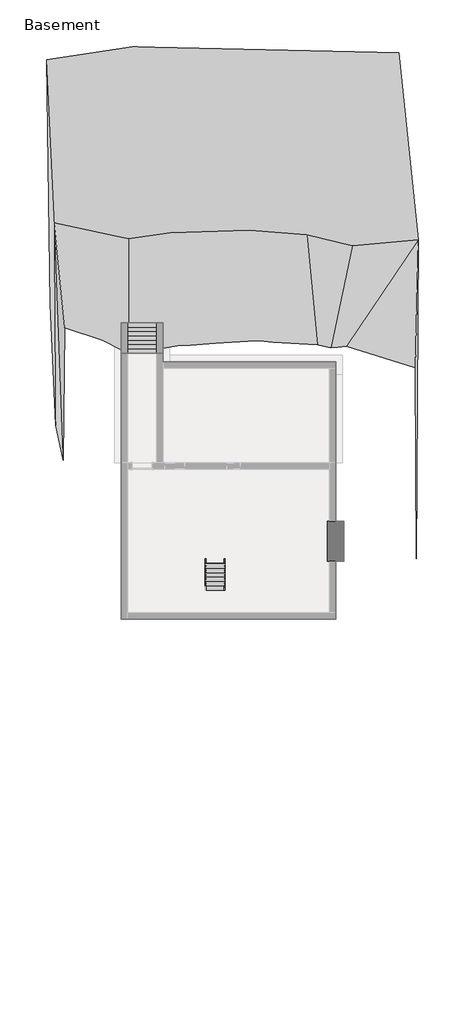
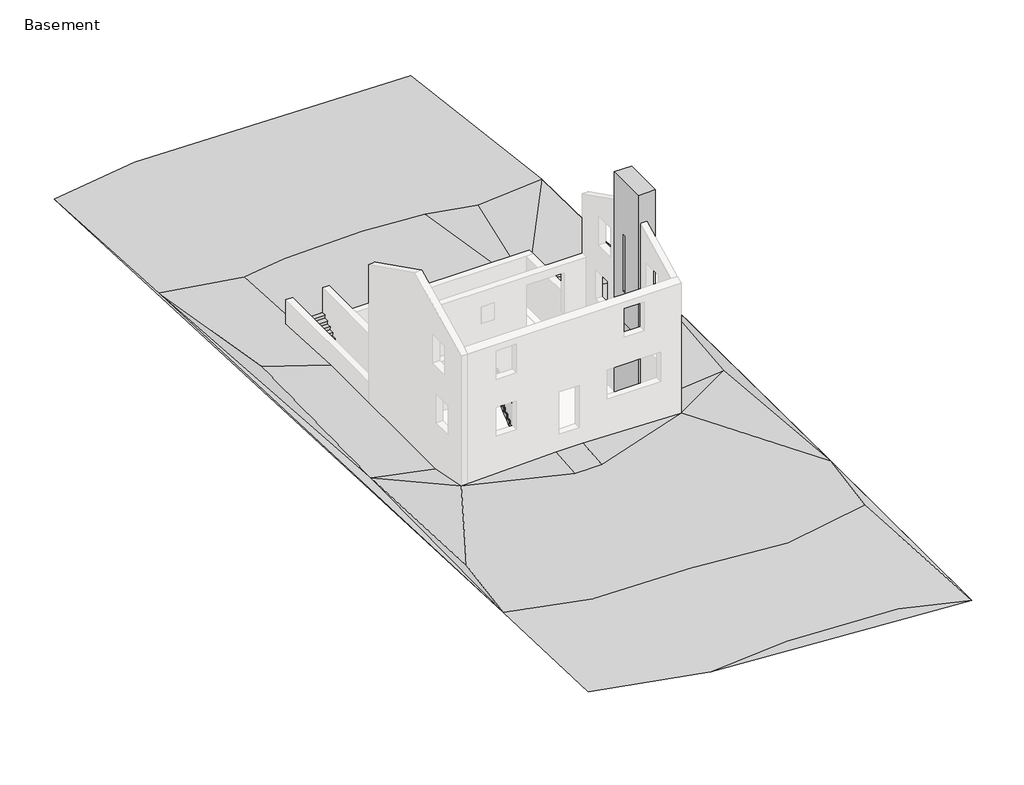
# One storey, part 2 of 2: 5 proxies, 2 members, 2 stair flights, 1 railing.
"""IFC4 building model written with IfcOpenShell, lengths in millimetres."""

import ifcopenshell
import ifcopenshell.guid

model = None  # the IFC model being written
_history = None  # IfcOwnerHistory: only IFC2X3 demands one
_inside = {}  # id of a spatial element -> (the spatial element, [elements in it])
_under = {}  # id of a project, library or spatial element -> (it, [spatial elements below it])
_declared = {}  # id of a project -> (the project, [libraries it declares])
_typed = {}  # id of a type object -> (the type object, [elements of that type])
_made_of = {}  # id of a material, layer set ... -> (it, [elements and type objects made of it])


def new_model(schema):
    """Start an empty IFC model of exactly this schema.

    Asked for "IFC4X3", IfcOpenShell would pick the latest addendum, in which some entities
    have other attributes; the version numbers below select the first issue.
    IFC2X3 requires an IfcOwnerHistory on every rooted entity: one is made here for all.
    """
    global model, _history
    if schema == "IFC4X3":
        model = ifcopenshell.file(schema_version=(4, 3, 0, 0))
    else:
        model = ifcopenshell.file(schema=schema)
    _inside.clear()
    _under.clear()
    _declared.clear()
    _typed.clear()
    _made_of.clear()
    _history = None
    if model.schema == "IFC2X3":
        org = make("IfcOrganization", Name="unknown")
        user = make(
            "IfcPersonAndOrganization",
            ThePerson=make("IfcPerson", FamilyName="unknown"),
            TheOrganization=org,
        )
        app = make(
            "IfcApplication",
            ApplicationDeveloper=org,
            Version="unknown",
            ApplicationFullName="unknown",
            ApplicationIdentifier="unknown",
        )
        _history = make(
            "IfcOwnerHistory",
            OwningUser=user,
            OwningApplication=app,
            ChangeAction="ADDED",
            CreationDate=0,
        )
    return model


def make(cls, **values):
    """One entity of the class cls with the attributes given. An attribute that is None is left unset."""
    return model.create_entity(
        cls, **{name: value for name, value in values.items() if value is not None}
    )


def rooted(cls, **values):
    """An entity with a GlobalId (a new one), such as an element, a storey or a relation."""
    return make(cls, GlobalId=ifcopenshell.guid.new(), OwnerHistory=_history, **values)


def si_unit(unit_type, name, prefix=None):
    """IfcSIUnit, for example si_unit("LENGTHUNIT", "METRE", prefix="MILLI")."""
    return make("IfcSIUnit", UnitType=unit_type, Prefix=prefix, Name=name)


def assignment(units):
    """IfcUnitAssignment: the units of a project."""
    return None if units is None else make("IfcUnitAssignment", Units=units)


def point(xyz):
    """IfcCartesianPoint."""
    return None if xyz is None else make("IfcCartesianPoint", Coordinates=xyz)


def direction(xyz):
    """IfcDirection."""
    return None if xyz is None else make("IfcDirection", DirectionRatios=xyz)


def frame(location, z_axis=None, x_axis=None):
    """IfcAxis2Placement3D, a coordinate frame: its origin and axes. An axis left out is left unset."""
    return make(
        "IfcAxis2Placement3D",
        Location=point(location),
        Axis=direction(z_axis),
        RefDirection=direction(x_axis),
    )


def origin():
    """The frame at (0, 0, 0) with its axes left unset."""
    return frame((0.0, 0.0, 0.0))


def place(relative_to, where):
    """IfcLocalPlacement: puts the frame where relative to a parent placement (None: the world)."""
    return make(
        "IfcLocalPlacement", PlacementRelTo=relative_to, RelativePlacement=where
    )


def context(
    kind, dimensions, precision=None, world=None, true_north=None, identifier=None
):
    """IfcGeometricRepresentationContext, for example the 3D "Model" context."""
    return make(
        "IfcGeometricRepresentationContext",
        ContextIdentifier=identifier,
        ContextType=kind,
        CoordinateSpaceDimension=dimensions,
        Precision=precision,
        WorldCoordinateSystem=world,
        TrueNorth=true_north,
    )


def project(units=None, contexts=None):
    """IfcProject with its units and contexts."""
    return rooted(
        "IfcProject",
        Name="project",
        RepresentationContexts=contexts,
        UnitsInContext=assignment(units),
    )


def spatial(cls, under=None, at=None, **own):
    """A site, building, storey or space (cls), placed at a placement, below another one or the project."""
    s = rooted(cls, ObjectPlacement=at, **own)
    if under is not None:
        _under.setdefault(under.id(), (under, []))[1].append(s)
    return s


def polyline(points):
    """IfcPolyline through the points."""
    return make("IfcPolyline", Points=[point(p) for p in points])


def point_list(points):
    """IfcCartesianPointList2D or 3D."""
    cls = (
        "IfcCartesianPointList2D" if len(points[0]) == 2 else "IfcCartesianPointList3D"
    )
    return make(cls, CoordList=points)


def outline(outer, holes=None, kind="AREA"):
    """IfcArbitraryClosedProfileDef: a profile drawn as a closed curve; with holes, ...WithVoids."""
    if holes is None:
        return make("IfcArbitraryClosedProfileDef", ProfileType=kind, OuterCurve=outer)
    return make(
        "IfcArbitraryProfileDefWithVoids",
        ProfileType=kind,
        OuterCurve=outer,
        InnerCurves=holes,
    )


def extrude(swept, where, along, depth):
    """IfcExtrudedAreaSolid: the profile swept, set in the frame where, extruded along a direction by depth."""
    return make(
        "IfcExtrudedAreaSolid",
        SweptArea=swept,
        Position=where,
        ExtrudedDirection=direction(along),
        Depth=depth,
    )


def faces_of(points, faces, orient=None, outer=None):
    """IfcFace entities. A face is a list of loops; a loop is a list of indices into points, from 0.

    orient and outer hold one flag for each loop. By default every Orientation is true, the
    first loop of a face is its IfcFaceOuterBound and the others are IfcFaceBound.
    """
    made = []
    for i, loops in enumerate(faces):
        bounds = []
        for j, loop in enumerate(loops):
            is_outer = j == 0 if outer is None else outer[i][j]
            bounds.append(
                make(
                    "IfcFaceOuterBound" if is_outer else "IfcFaceBound",
                    Bound=make("IfcPolyLoop", Polygon=[points[k] for k in loop]),
                    Orientation=True if orient is None else orient[i][j],
                )
            )
        made.append(make("IfcFace", Bounds=bounds))
    return made


def faceted_brep(points, faces, orient=None, outer=None, voids=None):
    """IfcFacetedBrep: a solid bounded by flat faces; with voids (closed shells), ...WithVoids."""
    shared = [point(p) for p in points]
    hull = make("IfcClosedShell", CfsFaces=faces_of(shared, faces, orient, outer))
    if voids is None:
        return make("IfcFacetedBrep", Outer=hull)
    return make(
        "IfcFacetedBrepWithVoids",
        Outer=hull,
        Voids=[
            make(cls, CfsFaces=faces_of(shared, fs, o, b)) for cls, fs, o, b in voids
        ],
    )


def triangles(points, corners, closed=None, point_numbers=None):
    """IfcTriangulatedFaceSet: each triangle names its three corners, points numbered from 1."""
    return make(
        "IfcTriangulatedFaceSet",
        Coordinates=point_list(points),
        Closed=closed,
        CoordIndex=corners,
        PnIndex=point_numbers,
    )


def shape(context_of_items, identifier, shape_type, items):
    """IfcShapeRepresentation: the items that make up one representation, for example the "Body"."""
    return make(
        "IfcShapeRepresentation",
        ContextOfItems=context_of_items,
        RepresentationIdentifier=identifier,
        RepresentationType=shape_type,
        Items=items,
    )


def source(mapping_origin, context_of_items, identifier, shape_type, items):
    """IfcRepresentationMap: a shape defined once, which mapped items show again and again."""
    return make(
        "IfcRepresentationMap",
        MappingOrigin=mapping_origin,
        MappedRepresentation=shape(context_of_items, identifier, shape_type, items),
    )


def transform(
    local_origin,
    x_axis=None,
    y_axis=None,
    z_axis=None,
    scale=None,
    scale2=None,
    scale3=None,
    uniform=True,
):
    """IfcCartesianTransformationOperator3D, or its non-uniform kind. x_axis, y_axis, z_axis: its Axis1, 2, 3."""
    if uniform:
        return make(
            "IfcCartesianTransformationOperator3D",
            Axis1=direction(x_axis),
            Axis2=direction(y_axis),
            LocalOrigin=point(local_origin),
            Scale=scale,
            Axis3=direction(z_axis),
        )
    return make(
        "IfcCartesianTransformationOperator3DnonUniform",
        Axis1=direction(x_axis),
        Axis2=direction(y_axis),
        LocalOrigin=point(local_origin),
        Scale=scale,
        Axis3=direction(z_axis),
        Scale2=scale2,
        Scale3=scale3,
    )


def mapped(mapping_source, mapping_target):
    """IfcMappedItem: shows the shape of a source again, moved by a transform."""
    return make(
        "IfcMappedItem", MappingSource=mapping_source, MappingTarget=mapping_target
    )


def made_of(thing, what):
    """Note that an element or type object is made of a material, layer set ...; save() writes the relation."""
    if what is not None:
        _made_of.setdefault(what.id(), (what, []))[1].append(thing)
    return thing


def element(
    cls,
    number,
    at=None,
    inside=None,
    cuts=None,
    type_object=None,
    material=None,
    context=None,
    identifier="Body",
    shape_type=None,
    held_by="IfcProductDefinitionShape",
    body=None,
    shapes=None,
    **own,
):
    """One element of the class cls, such as IfcWall. Its Tag is "e" and its number.

    at: its placement. inside: the storey or other place that contains it. cuts: it is an
    opening in that element (IfcRelVoidsElement). A single representation is given by context,
    identifier, shape_type and body (its items); several are given by shapes. held_by: the class
    of the entity that holds the representations. save() writes the other relations.
    """
    e = rooted(cls, Tag="e%d" % number, ObjectPlacement=at, **own)
    if body is not None:
        shapes = [shape(context, identifier, shape_type, body)]
    if shapes is not None:
        e.Representation = make(held_by, Representations=shapes)
    if inside is not None:
        _inside.setdefault(inside.id(), (inside, []))[1].append(e)
    if cuts is not None:
        rooted(
            "IfcRelVoidsElement", RelatingBuildingElement=cuts, RelatedOpeningElement=e
        )
    if type_object is not None:
        _typed.setdefault(type_object.id(), (type_object, []))[1].append(e)
    return made_of(e, material)


def aggregate(whole, parts):
    """IfcRelAggregates: a whole, such as a stair, and the parts it consists of."""
    return rooted("IfcRelAggregates", RelatingObject=whole, RelatedObjects=parts)


def save(model, path):
    """Write the relations noted so far, then the file.

    IfcRelAggregates (storeys below a building ...), IfcRelContainedInSpatialStructure (elements
    in a storey), IfcRelDefinesByType, IfcRelAssociatesMaterial and IfcRelDeclares: one each for
    every whole, place, type object, material and project.
    """
    for whole, parts in _under.values():
        aggregate(whole, parts)
    for where, things in _inside.values():
        rooted(
            "IfcRelContainedInSpatialStructure",
            RelatedElements=things,
            RelatingStructure=where,
        )
    for kind, things in _typed.values():
        rooted("IfcRelDefinesByType", RelatedObjects=things, RelatingType=kind)
    for what, things in _made_of.values():
        rooted("IfcRelAssociatesMaterial", RelatedObjects=things, RelatingMaterial=what)
    for by, libraries in _declared.values():
        rooted("IfcRelDeclares", RelatingContext=by, RelatedDefinitions=libraries)
    model.write(path)


def existing_fireplace_existing_fireplace_287aed51(model_context):
    return source(origin(), model_context, "Body", "Brep", [
        faceted_brep([(4450.2196932, 434.2888758, 8077.2), (3662.8196932, 434.2888758, 8077.2), (3662.8196932, -1445.3111242, 8077.2), (4450.2196932, -1445.3111242, 8077.2), (4450.2196932, 434.2888758, -2667.0), (4450.2196932, -1445.3111242, -2667.0), (4069.2196932, -1445.3111242, -2667.0), (3764.4196932, -1445.3111242, -2667.0), (3662.8196932, -1445.3111242, -2667.0), (3662.8196932, 434.2888758, -2667.0), (3764.4196932, 434.2888758, -2667.0), (4069.2196932, 434.2888758, -2667.0), (3662.8196932, 154.8888758, 0.0), (3662.8196932, 154.8888758, 1219.2), (3662.8196932, -1165.9111242, 1219.2), (3662.8196932, -1165.9111242, 0.0), (3662.8196932, -403.9111242, 5486.4), (3662.8196932, -403.9111242, 2743.2), (3662.8196932, -276.9111242, 2743.2), (3662.8196932, -276.9111242, 5486.4), (4145.4196932, -20.7631592, 1219.2), (4145.4196932, -990.2590891, 1219.2), (4145.4196932, -990.2590891, 0.0), (4145.4196932, -20.7631592, 0.0), (3767.2567114, -403.9111242, 5486.4), (3767.2567114, -403.9111242, 2743.2), (3767.2567114, -276.9111242, 2743.2), (3767.2567114, -276.9111242, 5486.4)], [[[0, 1, 2, 3]], [[4, 5, 6, 7, 8, 9, 10, 11]], [[1, 0, 4, 11, 10, 9]], [[2, 1, 9, 8], [12, 13, 14, 15], [16, 17, 18, 19]], [[3, 2, 8, 7, 6, 5]], [[0, 3, 5, 4]], [[14, 13, 20, 21]], [[15, 14, 21, 22]], [[21, 20, 23, 22]], [[13, 12, 23, 20]], [[12, 15, 22, 23]], [[24, 25, 17, 16]], [[26, 27, 19, 18]], [[25, 26, 18, 17]], [[25, 24, 27, 26]], [[27, 24, 16, 19]]]),
    ])


def stair_flight_b746b64e(model_context):
    return source(origin(), model_context, "Body", "SweptSolid", [
        extrude(outline(polyline([(-2791.5111242, -2476.5), (-2562.9111242, -2476.5), (-2562.9111242, -2527.3), (-2766.1111242, -2527.3), (-2766.1111242, -2520.95), (-2791.5111242, -2495.55), (-2791.5111242, -2476.5)])), frame((-2052.1803068, 0.0, 0.0), z_axis=(1.0, 0.0, 0.0), x_axis=(0.0, 1.0, 0.0)), (0.0, 0.0, 1.0), 939.8),
        extrude(outline(polyline([(-1112.3803068, -2759.7611242), (-1112.3803068, -2766.1111242), (-2052.1803068, -2766.1111242), (-2052.1803068, -2759.7611242), (-1112.3803068, -2759.7611242)])), frame((0.0, 0.0, -2667.0), z_axis=(0.0, 0.0, 1.0), x_axis=(1.0, 0.0, 0.0)), (0.0, 0.0, 1.0), 139.7),
        extrude(outline(polyline([(-1112.3803068, -2556.5611242), (-1112.3803068, -2562.9111242), (-2052.1803068, -2562.9111242), (-2052.1803068, -2556.5611242), (-1112.3803068, -2556.5611242)])), frame((0.0, 0.0, -2527.3), z_axis=(0.0, 0.0, 1.0), x_axis=(1.0, 0.0, 0.0)), (0.0, 0.0, 1.0), 190.5),
        extrude(outline(polyline([(-2588.3111242, -2286.0), (-2359.7111242, -2286.0), (-2359.7111242, -2336.8), (-2562.9111242, -2336.8), (-2562.9111242, -2330.45), (-2588.3111242, -2305.05), (-2588.3111242, -2286.0)])), frame((-2052.1803068, 0.0, 0.0), z_axis=(1.0, 0.0, 0.0), x_axis=(0.0, 1.0, 0.0)), (0.0, 0.0, 1.0), 939.8),
        extrude(outline(polyline([(-1112.3803068, -2353.3611242), (-1112.3803068, -2359.7111242), (-2052.1803068, -2359.7111242), (-2052.1803068, -2353.3611242), (-1112.3803068, -2353.3611242)])), frame((0.0, 0.0, -2336.8), z_axis=(0.0, 0.0, 1.0), x_axis=(1.0, 0.0, 0.0)), (0.0, 0.0, 1.0), 190.5),
        extrude(outline(polyline([(-2385.1111242, -2095.5), (-2156.5111242, -2095.5), (-2156.5111242, -2146.3), (-2359.7111242, -2146.3), (-2359.7111242, -2139.95), (-2385.1111242, -2114.55), (-2385.1111242, -2095.5)])), frame((-2052.1803068, 0.0, 0.0), z_axis=(1.0, 0.0, 0.0), x_axis=(0.0, 1.0, 0.0)), (0.0, 0.0, 1.0), 939.8),
        extrude(outline(polyline([(-1112.3803068, -2150.1611242), (-1112.3803068, -2156.5111242), (-2052.1803068, -2156.5111242), (-2052.1803068, -2150.1611242), (-1112.3803068, -2150.1611242)])), frame((0.0, 0.0, -2146.3), z_axis=(0.0, 0.0, 1.0), x_axis=(1.0, 0.0, 0.0)), (0.0, 0.0, 1.0), 190.5),
        extrude(outline(polyline([(-2181.9111242, -1905.0), (-1953.3111242, -1905.0), (-1953.3111242, -1955.8), (-2156.5111242, -1955.8), (-2156.5111242, -1949.45), (-2181.9111242, -1924.05), (-2181.9111242, -1905.0)])), frame((-2052.1803068, 0.0, 0.0), z_axis=(1.0, 0.0, 0.0), x_axis=(0.0, 1.0, 0.0)), (0.0, 0.0, 1.0), 939.8),
        extrude(outline(polyline([(-1112.3803068, -1946.9611242), (-1112.3803068, -1953.3111242), (-2052.1803068, -1953.3111242), (-2052.1803068, -1946.9611242), (-1112.3803068, -1946.9611242)])), frame((0.0, 0.0, -1955.8), z_axis=(0.0, 0.0, 1.0), x_axis=(1.0, 0.0, 0.0)), (0.0, 0.0, 1.0), 190.5),
        extrude(outline(polyline([(-1978.7111242, -1714.5), (-1750.1111242, -1714.5), (-1750.1111242, -1765.3), (-1953.3111242, -1765.3), (-1953.3111242, -1758.95), (-1978.7111242, -1733.55), (-1978.7111242, -1714.5)])), frame((-2052.1803068, 0.0, 0.0), z_axis=(1.0, 0.0, 0.0), x_axis=(0.0, 1.0, 0.0)), (0.0, 0.0, 1.0), 939.8),
        extrude(outline(polyline([(-1112.3803068, -1743.7611242), (-1112.3803068, -1750.1111242), (-2052.1803068, -1750.1111242), (-2052.1803068, -1743.7611242), (-1112.3803068, -1743.7611242)])), frame((0.0, 0.0, -1765.3), z_axis=(0.0, 0.0, 1.0), x_axis=(1.0, 0.0, 0.0)), (0.0, 0.0, 1.0), 190.5),
        extrude(outline(polyline([(-1775.5111242, -1524.0), (-1546.9111242, -1524.0), (-1546.9111242, -1574.8), (-1750.1111242, -1574.8), (-1750.1111242, -1568.45), (-1775.5111242, -1543.05), (-1775.5111242, -1524.0)])), frame((-2052.1803068, 0.0, 0.0), z_axis=(1.0, 0.0, 0.0), x_axis=(0.0, 1.0, 0.0)), (0.0, 0.0, 1.0), 939.8),
        extrude(outline(polyline([(-1112.3803068, -1540.5611242), (-1112.3803068, -1546.9111242), (-2052.1803068, -1546.9111242), (-2052.1803068, -1540.5611242), (-1112.3803068, -1540.5611242)])), frame((0.0, 0.0, -1574.8), z_axis=(0.0, 0.0, 1.0), x_axis=(1.0, 0.0, 0.0)), (0.0, 0.0, 1.0), 190.5),
        extrude(outline(polyline([(-1572.3111242, -1333.5), (-1343.7111242, -1333.5), (-1343.7111242, -1384.3), (-1546.9111242, -1384.3), (-1546.9111242, -1377.95), (-1572.3111242, -1352.55), (-1572.3111242, -1333.5)])), frame((-2052.1803068, 0.0, 0.0), z_axis=(1.0, 0.0, 0.0), x_axis=(0.0, 1.0, 0.0)), (0.0, 0.0, 1.0), 939.8),
        extrude(outline(polyline([(-1112.3803068, -1337.3611242), (-1112.3803068, -1343.7111242), (-2052.1803068, -1343.7111242), (-2052.1803068, -1337.3611242), (-1112.3803068, -1337.3611242)])), frame((0.0, 0.0, -1384.3), z_axis=(0.0, 0.0, 1.0), x_axis=(1.0, 0.0, 0.0)), (0.0, 0.0, 1.0), 190.5),
        extrude(outline(polyline([(-1369.1111242, -1143.0), (-1140.5111242, -1143.0), (-1140.5111242, -1193.8), (-1343.7111242, -1193.8), (-1343.7111242, -1187.45), (-1369.1111242, -1162.05), (-1369.1111242, -1143.0)])), frame((-2052.1803068, 0.0, 0.0), z_axis=(1.0, 0.0, 0.0), x_axis=(0.0, 1.0, 0.0)), (0.0, 0.0, 1.0), 939.8),
        extrude(outline(polyline([(-1112.3803068, -1134.1611242), (-1112.3803068, -1140.5111242), (-2052.1803068, -1140.5111242), (-2052.1803068, -1134.1611242), (-1112.3803068, -1134.1611242)])), frame((0.0, 0.0, -1193.8), z_axis=(0.0, 0.0, 1.0), x_axis=(1.0, 0.0, 0.0)), (0.0, 0.0, 1.0), 190.5),
        extrude(outline(polyline([(-1165.9111242, -952.5), (-937.3111242, -952.5), (-937.3111242, -1003.3), (-1140.5111242, -1003.3), (-1140.5111242, -996.95), (-1165.9111242, -971.55), (-1165.9111242, -952.5)])), frame((-2052.1803068, 0.0, 0.0), z_axis=(1.0, 0.0, 0.0), x_axis=(0.0, 1.0, 0.0)), (0.0, 0.0, 1.0), 939.8),
        extrude(outline(polyline([(-1112.3803068, -930.9611242), (-1112.3803068, -937.3111242), (-2052.1803068, -937.3111242), (-2052.1803068, -930.9611242), (-1112.3803068, -930.9611242)])), frame((0.0, 0.0, -1003.3), z_axis=(0.0, 0.0, 1.0), x_axis=(1.0, 0.0, 0.0)), (0.0, 0.0, 1.0), 190.5),
        extrude(outline(polyline([(-962.7111242, -762.0), (-734.1111242, -762.0), (-734.1111242, -812.8), (-937.3111242, -812.8), (-937.3111242, -806.45), (-962.7111242, -781.05), (-962.7111242, -762.0)])), frame((-2052.1803068, 0.0, 0.0), z_axis=(1.0, 0.0, 0.0), x_axis=(0.0, 1.0, 0.0)), (0.0, 0.0, 1.0), 939.8),
        extrude(outline(polyline([(-1112.3803068, -727.7611242), (-1112.3803068, -734.1111242), (-2052.1803068, -734.1111242), (-2052.1803068, -727.7611242), (-1112.3803068, -727.7611242)])), frame((0.0, 0.0, -812.8), z_axis=(0.0, 0.0, 1.0), x_axis=(1.0, 0.0, 0.0)), (0.0, 0.0, 1.0), 190.5),
        extrude(outline(polyline([(-759.5111242, -571.5), (-530.9111242, -571.5), (-530.9111242, -622.3), (-734.1111242, -622.3), (-734.1111242, -615.95), (-759.5111242, -590.55), (-759.5111242, -571.5)])), frame((-2052.1803068, 0.0, 0.0), z_axis=(1.0, 0.0, 0.0), x_axis=(0.0, 1.0, 0.0)), (0.0, 0.0, 1.0), 939.8),
        extrude(outline(polyline([(-1112.3803068, -524.5611242), (-1112.3803068, -530.9111242), (-2052.1803068, -530.9111242), (-2052.1803068, -524.5611242), (-1112.3803068, -524.5611242)])), frame((0.0, 0.0, -622.3), z_axis=(0.0, 0.0, 1.0), x_axis=(1.0, 0.0, 0.0)), (0.0, 0.0, 1.0), 190.5),
        extrude(outline(polyline([(-556.3111242, -381.0), (-327.7111242, -381.0), (-327.7111242, -431.8), (-530.9111242, -431.8), (-530.9111242, -425.45), (-556.3111242, -400.05), (-556.3111242, -381.0)])), frame((-2052.1803068, 0.0, 0.0), z_axis=(1.0, 0.0, 0.0), x_axis=(0.0, 1.0, 0.0)), (0.0, 0.0, 1.0), 939.8),
        extrude(outline(polyline([(-1112.3803068, -321.3611242), (-1112.3803068, -327.7111242), (-2052.1803068, -327.7111242), (-2052.1803068, -321.3611242), (-1112.3803068, -321.3611242)])), frame((0.0, 0.0, -431.8), z_axis=(0.0, 0.0, 1.0), x_axis=(1.0, 0.0, 0.0)), (0.0, 0.0, 1.0), 190.5),
        extrude(outline(polyline([(-353.1111242, -190.5), (-124.5111242, -190.5), (-124.5111242, -241.3), (-327.7111242, -241.3), (-327.7111242, -234.95), (-353.1111242, -209.55), (-353.1111242, -190.5)])), frame((-2052.1803068, 0.0, 0.0), z_axis=(1.0, 0.0, 0.0), x_axis=(0.0, 1.0, 0.0)), (0.0, 0.0, 1.0), 939.8),
        extrude(outline(polyline([(-1112.3803068, -118.1611242), (-1112.3803068, -124.5111242), (-2052.1803068, -124.5111242), (-2052.1803068, -118.1611242), (-1112.3803068, -118.1611242)])), frame((0.0, 0.0, -241.3), z_axis=(0.0, 0.0, 1.0), x_axis=(1.0, 0.0, 0.0)), (0.0, 0.0, 1.0), 190.5),
    ])


model = new_model("IFC4")

# Units and contexts
model_context = context("Model", 3, world=origin())
ifc_project = project(units=[si_unit("LENGTHUNIT", "METRE", prefix="MILLI")], contexts=[model_context])

# Site, building, storey
site = spatial("IfcSite", under=ifc_project)
building = spatial("IfcBuilding", under=site)
storey = spatial("IfcBuildingStorey", under=building, Name="Basement", Elevation=-2667.0)

# Proxies
placement = place(None, origin())
element("IfcBuildingElementProxy", 1, Name="Building Element Proxy", at=placement, inside=storey, context=model_context, shape_type="Tessellation", body=[
    triangles([(-9474.14729, 22003.2871765, -1727.1999516), (-8916.1412338, -12566.1132111, -939.7999758), (-8632.7724838, -18803.3999359, -1092.1999758), (-3754.3850807, -20036.8885986, -1092.1999758), (7677.2023224, -20906.8378235, -1092.1999758), (7936.7585724, 13587.9496765, -1752.6), (7012.0400162, 22339.8364014, -1727.1999516), (-5437.1349838, 22620.8239014, -1727.1999516), (-5989.1803574, 9705.2889954, -1534.1892036), (-5618.9576065, 9705.2889954, -1544.3833488), (-4007.9803574, 9705.2889954, -1530.2029644), (-4007.9803574, 8275.4099945, -1454.6497272), (-4007.9803574, 7876.4889954, -1433.5712173), (-2888.427182, 7876.4889954, -1423.716441), (-2503.8244949, 7876.4889954, -1420.7760681), (-1830.9343174, 7876.4889954, -1419.6736645), (382.6070967, 7876.4889954, -1412.0516006), (830.4323782, 7876.4889954, -1414.120079), (3292.100798, 7876.4889954, -1421.9283234), (3708.8884392, 7876.4889954, -1427.5587936), (4069.2196426, 7876.4889954, -1425.5557182), (4069.2196426, 7529.9159637, -1404.4058464), (4069.2196426, 6299.0253983, -1346.1999516), (4069.2196426, 3152.0889954, -1346.1999516), (4069.2196426, 434.2888621, -1346.1999516), (4450.2196426, 434.2888621, -1346.1999516), (4450.2196426, -349.5066825, -1346.1999516), (4450.2196426, -1445.3110531, -1346.1999516), (4069.2196426, -1445.3110531, -1346.1999516), (4069.2196426, -2313.9084709, -1346.1999516), (4069.2196426, -4163.1110046, -939.7999758), (-426.580321, -4163.1110046, -812.8000242), (-1645.7803574, -4163.1110046, -812.8000242), (-5989.1803574, -4163.1110046, -939.7999758), (-5989.1803574, -2124.4043404, -1346.1999516), (-5989.1803574, 3152.0889954, -1346.1999516), (-5989.1803574, 4989.0600082, -1346.1999516), (-5989.1803574, 6156.3282944, -1346.1999516), (-5989.1803574, 8275.4099945, -1458.4483326), (-9109.81604, 14372.1750641, -1752.6), (-8549.4287338, -9013.2876297, -939.7999758), (-8523.2349838, -1401.2252266, -1346.1999516), (-8408.9349838, 7414.1625641, -1346.1999516), (-6082.4537338, -10022.9382111, -939.7999758), (-5633.19104, 13643.5125641, -1752.6), (-5382.3662338, -13518.6132111, -939.7999758), (-3671.0413307, 13924.5000641, -1752.6), (-2942.3788307, -9965.7882111, -939.7999758), (-1568.3975807, 21947.7254517, -1727.1999516), (-840.5287823, -13629.7378235, -939.7999758), (-699.241258, -10470.6132111, -939.7999758), (-109.4850414, -19700.3370483, -1092.1999758), (29.4212079, 14035.6246765, -1752.6), (2721.8210724, 13811.7871765, -1752.6), (2805.1648224, 21892.1614014, -1727.1999516), (3252.0462662, -14021.8499359, -939.7999758), (4179.1460724, -9854.6624359, -939.7999758), (4845.1025162, -19962.2745483, -1092.1999758), (4852.2462662, 13306.9621765, -1752.6), (7177.93396, -13294.7757111, -939.7999758), (7289.85271, -1961.6126781, -1346.1999516), (7543.0587662, -9965.7882111, -939.7999758), (7740.7025162, 5059.8998703, -1346.1999516), (-1645.7803574, -5668.0610046, -939.7999758), (-426.580321, -5668.0610046, -939.7999758)], [[44, 2, 46], [41, 44, 34], [44, 41, 2], [2, 3, 46], [2, 41, 42], [43, 37, 38], [36, 37, 43], [43, 42, 36], [35, 42, 34], [42, 41, 34], [44, 64, 34], [2, 42, 40], [46, 4, 50], [4, 46, 3], [64, 48, 51], [50, 48, 46], [4, 52, 50], [64, 44, 48], [35, 36, 42], [65, 33, 64], [64, 33, 34], [48, 44, 46], [43, 9, 40], [9, 43, 39], [38, 39, 43], [9, 10, 45], [1, 40, 8], [40, 1, 2], [45, 8, 40], [47, 8, 45], [40, 9, 45], [45, 10, 11], [43, 40, 42], [12, 13, 14], [14, 15, 11], [16, 11, 15], [12, 14, 11], [47, 49, 8], [53, 47, 11], [53, 49, 47], [11, 47, 45], [16, 53, 11], [8, 49, 55], [48, 50, 51], [65, 32, 33], [57, 31, 65], [56, 51, 50], [56, 52, 58], [50, 52, 56], [51, 57, 65], [29, 30, 28], [32, 65, 31], [61, 30, 31], [51, 56, 57], [56, 60, 57], [60, 58, 5], [62, 5, 63], [5, 62, 60], [58, 52, 5], [57, 60, 62], [57, 62, 31], [28, 61, 27], [28, 30, 61], [62, 61, 31], [27, 61, 26], [62, 63, 61], [60, 56, 58], [52, 4, 5], [53, 17, 18], [54, 18, 19], [53, 54, 55], [53, 18, 54], [20, 59, 19], [54, 59, 55], [54, 19, 59], [53, 55, 49], [53, 16, 17], [23, 24, 63], [26, 63, 24], [63, 26, 61], [24, 25, 26], [23, 63, 22], [22, 63, 21], [59, 6, 7], [6, 59, 21], [59, 7, 55], [63, 6, 21], [21, 59, 20], [63, 5, 6], [55, 7, 8], [64, 51, 65]], closed=False),
])
element("IfcBuildingElementProxy", 2, Name="Building Element Proxy", at=placement, inside=storey, context=model_context, shape_type="Tessellation", body=[
    triangles([(4069.2196426, 3152.0889954, -3073.5594864), (4069.2196426, 3152.0889954, -1346.1999516), (4069.2196426, 434.2888621, -3073.5594864), (4069.2196426, 434.2888621, -1346.1999516), (4450.2196426, 434.2888621, -3073.5594864), (4450.2196426, 434.2888621, -1346.1999516), (4450.2196426, -349.5066825, -3073.5594864), (4450.2196426, -349.5066825, -1346.1999516), (4450.2196426, -1445.3110531, -3073.5594864), (4450.2196426, -1445.3110531, -1346.1999516), (4069.2196426, -1445.3110531, -3073.5594864), (4069.2196426, -1445.3110531, -1346.1999516), (4069.2196426, -2313.9084709, -3073.5594864), (4069.2196426, -2313.9084709, -1346.1999516), (4069.2196426, -4163.1110046, -3073.5594864), (4069.2196426, -4163.1110046, -939.7999758), (-426.580321, -4163.1110046, -3073.5594864), (-426.580321, -4163.1110046, -812.8000242), (-1645.7803574, -4163.1110046, -3073.5594864), (-1645.7803574, -4163.1110046, -812.8000242), (-5989.1803574, -4163.1110046, -3073.5594864), (-5989.1803574, -4163.1110046, -939.7999758), (-5989.1803574, -2124.4043404, -3073.5594864), (-5989.1803574, -2124.4043404, -1346.1999516), (-5989.1803574, 3152.0889954, -3073.5594864), (-5989.1803574, 3152.0889954, -1346.1999516)], [[1, 4, 2], [1, 3, 4], [3, 6, 4], [3, 5, 6], [5, 8, 6], [5, 7, 8], [7, 10, 8], [7, 9, 10], [9, 12, 10], [9, 11, 12], [11, 14, 12], [11, 13, 14], [13, 16, 14], [13, 15, 16], [15, 18, 16], [15, 17, 18], [17, 20, 18], [17, 19, 20], [19, 22, 20], [19, 21, 22], [21, 24, 22], [21, 23, 24], [23, 26, 24], [23, 25, 26]], closed=False),
    triangles([(4069.2196426, 434.2888621, -3073.5594864), (4069.2196426, 3152.0889954, -3073.5594864), (-5989.1803574, 3152.0889954, -3073.5594864), (-5989.1803574, -4163.1110046, -3073.5594864), (4069.2196426, -4163.1110046, -3073.5594864), (4069.2196426, -1445.3110531, -3073.5594864), (4450.2196426, -1445.3110531, -3073.5594864), (4450.2196426, 434.2888621, -3073.5594864)], [[4, 6, 3], [6, 4, 5], [3, 1, 2], [1, 3, 6], [6, 7, 1], [8, 1, 7]], closed=False),
])
element("IfcBuildingElementProxy", 3, Name="Building Element Proxy", at=placement, inside=storey, context=model_context, shape_type="Tessellation", body=[
    triangles([(4069.2196426, 3152.0889954, -3073.5594864), (4069.2196426, 3152.0889954, -1346.1999516), (4069.2196426, 6299.0253983, -3073.5594864), (4069.2196426, 6299.0253983, -1346.1999516), (4069.2196426, 7529.9159637, -3073.5594864), (4069.2196426, 7529.9159637, -1404.4058464), (4069.2196426, 7876.4889954, -3073.5594864), (4069.2196426, 7876.4889954, -1425.5557182), (3708.8884392, 7876.4889954, -3073.5594864), (3708.8884392, 7876.4889954, -1427.5587936), (3292.100798, 7876.4889954, -3073.5594864), (3292.100798, 7876.4889954, -1421.9283234), (830.4323782, 7876.4889954, -3073.5594864), (830.4323782, 7876.4889954, -1414.120079), (382.6070967, 7876.4889954, -3073.5594864), (382.6070967, 7876.4889954, -1412.0516006), (-1830.9343174, 7876.4889954, -3073.5594864), (-1830.9343174, 7876.4889954, -1419.6736645), (-2503.8244949, 7876.4889954, -3073.5594864), (-2503.8244949, 7876.4889954, -1420.7760681), (-2888.427182, 7876.4889954, -3073.5594864), (-2888.427182, 7876.4889954, -1423.716441), (-4007.9803574, 7876.4889954, -3073.5594864), (-4007.9803574, 7876.4889954, -1433.5712173), (-4007.9803574, 8275.4099945, -3073.5594864), (-4007.9803574, 8275.4099945, -1454.6497272)], [[1, 4, 2], [1, 3, 4], [3, 6, 4], [3, 5, 6], [5, 8, 6], [5, 7, 8], [7, 10, 8], [7, 9, 10], [9, 12, 10], [9, 11, 12], [11, 14, 12], [11, 13, 14], [13, 16, 14], [13, 15, 16], [15, 18, 16], [15, 17, 18], [17, 20, 18], [17, 19, 20], [19, 22, 20], [19, 21, 22], [21, 24, 22], [21, 23, 24], [23, 26, 24], [23, 25, 26]], closed=False),
    triangles([(-5989.1803574, 8275.4099945, -3073.5594864), (-5989.1803574, 8275.4099945, -1458.4483326), (-5989.1803574, 6156.3282944, -3073.5594864), (-5989.1803574, 6156.3282944, -1346.1999516), (-5989.1803574, 4989.0600082, -3073.5594864), (-5989.1803574, 4989.0600082, -1346.1999516), (-5989.1803574, 3152.0889954, -3073.5594864), (-5989.1803574, 3152.0889954, -1346.1999516)], [[1, 4, 2], [1, 3, 4], [3, 6, 4], [3, 5, 6], [5, 8, 6], [5, 7, 8]], closed=False),
    triangles([(-5989.1803574, 8275.4099945, -3073.5594864), (-5989.1803574, 3152.0889954, -3073.5594864), (4069.2196426, 3152.0889954, -3073.5594864), (4069.2196426, 7876.4889954, -3073.5594864), (-4007.9803574, 7876.4889954, -3073.5594864), (-4007.9803574, 8275.4099945, -3073.5594864)], [[6, 1, 5], [5, 1, 2], [5, 3, 4], [3, 5, 2]], closed=False),
])
element("IfcBuildingElementProxy", 4, Name="Building Element Proxy", at=placement, inside=storey, context=model_context, shape_type="Tessellation", body=[
    triangles([(-5989.1803574, 8275.4099945, -2776.675573), (-5989.1803574, 8275.4099945, -3073.5594864), (-5613.7898987, 8275.4099945, -2776.675573), (-5613.7898987, 8275.4099945, -3073.5594864), (-4007.9803574, 8275.4099945, -2776.675573), (-4007.9803574, 8275.4099945, -3073.5594864)], [[1, 4, 2], [1, 3, 4], [3, 6, 4], [3, 5, 6]], closed=False),
    triangles([(-5989.1803574, 8275.4099945, -2776.675573), (-5989.1803574, 8275.4099945, -1458.4483326), (-5989.1803574, 9705.2889954, -1653.2006893), (-5989.1803574, 9705.2889954, -1534.1892036), (-5618.9576065, 9705.2889954, -1653.2006893), (-5618.9576065, 9705.2889954, -1544.3833488), (-4007.9803574, 9705.2889954, -1653.2006893), (-4007.9803574, 9705.2889954, -1530.2029644), (-4007.9803574, 8275.4099945, -2776.675573), (-4007.9803574, 8275.4099945, -1454.6497272)], [[1, 4, 2], [1, 3, 4], [3, 6, 4], [3, 5, 6], [5, 8, 6], [5, 7, 8], [7, 10, 8], [7, 9, 10]], closed=False),
    triangles([(-5989.1803574, 9705.2889954, -1653.2006893), (-5989.1803574, 8275.4099945, -2776.675573), (-4007.9803574, 8275.4099945, -2776.675573), (-4007.9803574, 9705.2889954, -1653.2006893)], [[1, 2, 4], [3, 4, 2]], closed=False),
])
existing_fireplace_existing_fireplace_shape = existing_fireplace_existing_fireplace_287aed51(model_context)
element("IfcBuildingElementProxy", 5, Name="Existing Fireplace : Existing Fireplace", ObjectType="Existing Fireplace : Existing Fireplace", at=placement, inside=storey, context=model_context, shape_type="MappedRepresentation", body=[
    mapped(existing_fireplace_existing_fireplace_shape, transform((0.0, 0.0, 0.0), x_axis=(1.0, 0.0, 0.0), y_axis=(0.0, 1.0, 0.0), z_axis=(0.0, 0.0, 1.0))),
])

# Members
element("IfcMember", 6, at=placement, inside=storey, context=model_context, shape_type="Brep", body=[
    faceted_brep([(-2052.1803068, -2759.7611242, -2667.0), (-2052.1803068, -2612.7302092, -2667.0), (-2001.3803068, -2612.7302092, -2667.0), (-2001.3803068, -2759.7611242, -2667.0), (-2001.3803068, -149.9111242, -358.1071078), (-2052.1803068, -149.9111242, -358.1071078), (-2052.1803068, -149.9111242, -241.3), (-2001.3803068, -149.9111242, -241.3), (-2052.1803068, -2556.5611242, -2614.3414828), (-2052.1803068, -2353.3611242, -2423.8414828), (-2052.1803068, -2150.1611242, -2233.3414828), (-2052.1803068, -1946.9611242, -2042.8414828), (-2052.1803068, -1743.7611242, -1852.3414828), (-2052.1803068, -1540.5611242, -1661.8414828), (-2052.1803068, -1337.3611242, -1471.3414828), (-2052.1803068, -1134.1611242, -1280.8414828), (-2052.1803068, -930.9611242, -1090.3414828), (-2052.1803068, -727.7611242, -899.8414828), (-2052.1803068, -524.5611242, -709.3414828), (-2052.1803068, -321.3611242, -518.8414828), (-2052.1803068, -2759.7611242, -2527.3), (-2052.1803068, -2556.5611242, -2527.3), (-2052.1803068, -2556.5611242, -2336.8), (-2052.1803068, -2353.3611242, -2336.8), (-2052.1803068, -2353.3611242, -2146.3), (-2052.1803068, -2150.1611242, -2146.3), (-2052.1803068, -2150.1611242, -1955.8), (-2052.1803068, -1946.9611242, -1955.8), (-2052.1803068, -1946.9611242, -1765.3), (-2052.1803068, -1743.7611242, -1765.3), (-2052.1803068, -1743.7611242, -1574.8), (-2052.1803068, -1540.5611242, -1574.8), (-2052.1803068, -1540.5611242, -1384.3), (-2052.1803068, -1337.3611242, -1384.3), (-2052.1803068, -1337.3611242, -1193.8), (-2052.1803068, -1134.1611242, -1193.8), (-2052.1803068, -1134.1611242, -1003.3), (-2052.1803068, -930.9611242, -1003.3), (-2052.1803068, -930.9611242, -812.8), (-2052.1803068, -727.7611242, -812.8), (-2052.1803068, -727.7611242, -622.3), (-2052.1803068, -524.5611242, -622.3), (-2052.1803068, -524.5611242, -431.8), (-2052.1803068, -321.3611242, -431.8), (-2052.1803068, -321.3611242, -241.3), (-2001.3803068, -321.3611242, -241.3), (-2001.3803068, -321.3611242, -431.8), (-2001.3803068, -524.5611242, -431.8), (-2001.3803068, -524.5611242, -622.3), (-2001.3803068, -727.7611242, -622.3), (-2001.3803068, -727.7611242, -812.8), (-2001.3803068, -930.9611242, -812.8), (-2001.3803068, -930.9611242, -1003.3), (-2001.3803068, -1134.1611242, -1003.3), (-2001.3803068, -1134.1611242, -1193.8), (-2001.3803068, -1337.3611242, -1193.8), (-2001.3803068, -1337.3611242, -1384.3), (-2001.3803068, -1540.5611242, -1384.3), (-2001.3803068, -1540.5611242, -1574.8), (-2001.3803068, -1743.7611242, -1574.8), (-2001.3803068, -1743.7611242, -1765.3), (-2001.3803068, -1946.9611242, -1765.3), (-2001.3803068, -1946.9611242, -1955.8), (-2001.3803068, -2150.1611242, -1955.8), (-2001.3803068, -2150.1611242, -2146.3), (-2001.3803068, -2353.3611242, -2146.3), (-2001.3803068, -2353.3611242, -2336.8), (-2001.3803068, -2556.5611242, -2336.8), (-2001.3803068, -2556.5611242, -2527.3), (-2001.3803068, -2759.7611242, -2527.3)], [[[0, 1, 2, 3]], [[4, 5, 6, 7]], [[5, 4, 2, 1, 8, 9, 10, 11, 12, 13, 14, 15, 16, 17, 18, 19]], [[6, 5, 19, 18, 17, 16, 15, 14, 13, 12, 11, 10, 9, 8, 1, 0, 20, 21, 22, 23, 24, 25, 26, 27, 28, 29, 30, 31, 32, 33, 34, 35, 36, 37, 38, 39, 40, 41, 42, 43, 44]], [[44, 45, 7, 6]], [[4, 7, 45, 46, 47, 48, 49, 50, 51, 52, 53, 54, 55, 56, 57, 58, 59, 60, 61, 62, 63, 64, 65, 66, 67, 68, 69, 3, 2]], [[69, 20, 0, 3]], [[20, 69, 68, 21]], [[21, 68, 67, 22]], [[22, 67, 66, 23]], [[23, 66, 65, 24]], [[24, 65, 64, 25]], [[25, 64, 63, 26]], [[26, 63, 62, 27]], [[27, 62, 61, 28]], [[28, 61, 60, 29]], [[29, 60, 59, 30]], [[30, 59, 58, 31]], [[31, 58, 57, 32]], [[32, 57, 56, 33]], [[33, 56, 55, 34]], [[34, 55, 54, 35]], [[35, 54, 53, 36]], [[36, 53, 52, 37]], [[37, 52, 51, 38]], [[38, 51, 50, 39]], [[39, 50, 49, 40]], [[40, 49, 48, 41]], [[41, 48, 47, 42]], [[42, 47, 46, 43]], [[43, 46, 45, 44]]]),
])
element("IfcMember", 7, at=placement, inside=storey, context=model_context, shape_type="Brep", body=[
    faceted_brep([(-1163.1803068, -2759.7611242, -2667.0), (-1163.1803068, -2612.7302092, -2667.0), (-1112.3803068, -2612.7302092, -2667.0), (-1112.3803068, -2759.7611242, -2667.0), (-1112.3803068, -149.9111242, -358.1071078), (-1163.1803068, -149.9111242, -358.1071078), (-1163.1803068, -149.9111242, -241.3), (-1112.3803068, -149.9111242, -241.3), (-1112.3803068, -321.3611242, -518.8414828), (-1112.3803068, -524.5611242, -709.3414828), (-1112.3803068, -727.7611242, -899.8414828), (-1112.3803068, -930.9611242, -1090.3414828), (-1112.3803068, -1134.1611242, -1280.8414828), (-1112.3803068, -1337.3611242, -1471.3414828), (-1112.3803068, -1540.5611242, -1661.8414828), (-1112.3803068, -1743.7611242, -1852.3414828), (-1112.3803068, -1946.9611242, -2042.8414828), (-1112.3803068, -2150.1611242, -2233.3414828), (-1112.3803068, -2353.3611242, -2423.8414828), (-1112.3803068, -2556.5611242, -2614.3414828), (-1163.1803068, -2759.7611242, -2527.3), (-1163.1803068, -2556.5611242, -2527.3), (-1163.1803068, -2556.5611242, -2336.8), (-1163.1803068, -2353.3611242, -2336.8), (-1163.1803068, -2353.3611242, -2146.3), (-1163.1803068, -2150.1611242, -2146.3), (-1163.1803068, -2150.1611242, -1955.8), (-1163.1803068, -1946.9611242, -1955.8), (-1163.1803068, -1946.9611242, -1765.3), (-1163.1803068, -1743.7611242, -1765.3), (-1163.1803068, -1743.7611242, -1574.8), (-1163.1803068, -1540.5611242, -1574.8), (-1163.1803068, -1540.5611242, -1384.3), (-1163.1803068, -1337.3611242, -1384.3), (-1163.1803068, -1337.3611242, -1193.8), (-1163.1803068, -1134.1611242, -1193.8), (-1163.1803068, -1134.1611242, -1003.3), (-1163.1803068, -930.9611242, -1003.3), (-1163.1803068, -930.9611242, -812.8), (-1163.1803068, -727.7611242, -812.8), (-1163.1803068, -727.7611242, -622.3), (-1163.1803068, -524.5611242, -622.3), (-1163.1803068, -524.5611242, -431.8), (-1163.1803068, -321.3611242, -431.8), (-1163.1803068, -321.3611242, -241.3), (-1112.3803068, -321.3611242, -241.3), (-1112.3803068, -321.3611242, -431.8), (-1112.3803068, -524.5611242, -431.8), (-1112.3803068, -524.5611242, -622.3), (-1112.3803068, -727.7611242, -622.3), (-1112.3803068, -727.7611242, -812.8), (-1112.3803068, -930.9611242, -812.8), (-1112.3803068, -930.9611242, -1003.3), (-1112.3803068, -1134.1611242, -1003.3), (-1112.3803068, -1134.1611242, -1193.8), (-1112.3803068, -1337.3611242, -1193.8), (-1112.3803068, -1337.3611242, -1384.3), (-1112.3803068, -1540.5611242, -1384.3), (-1112.3803068, -1540.5611242, -1574.8), (-1112.3803068, -1743.7611242, -1574.8), (-1112.3803068, -1743.7611242, -1765.3), (-1112.3803068, -1946.9611242, -1765.3), (-1112.3803068, -1946.9611242, -1955.8), (-1112.3803068, -2150.1611242, -1955.8), (-1112.3803068, -2150.1611242, -2146.3), (-1112.3803068, -2353.3611242, -2146.3), (-1112.3803068, -2353.3611242, -2336.8), (-1112.3803068, -2556.5611242, -2336.8), (-1112.3803068, -2556.5611242, -2527.3), (-1112.3803068, -2759.7611242, -2527.3)], [[[0, 1, 2, 3]], [[4, 5, 6, 7]], [[5, 4, 8, 9, 10, 11, 12, 13, 14, 15, 16, 17, 18, 19, 2, 1]], [[6, 5, 1, 0, 20, 21, 22, 23, 24, 25, 26, 27, 28, 29, 30, 31, 32, 33, 34, 35, 36, 37, 38, 39, 40, 41, 42, 43, 44]], [[44, 45, 7, 6]], [[4, 7, 45, 46, 47, 48, 49, 50, 51, 52, 53, 54, 55, 56, 57, 58, 59, 60, 61, 62, 63, 64, 65, 66, 67, 68, 69, 3, 2, 19, 18, 17, 16, 15, 14, 13, 12, 11, 10, 9, 8]], [[69, 20, 0, 3]], [[20, 69, 68, 21]], [[21, 68, 67, 22]], [[22, 67, 66, 23]], [[23, 66, 65, 24]], [[24, 65, 64, 25]], [[25, 64, 63, 26]], [[26, 63, 62, 27]], [[27, 62, 61, 28]], [[28, 61, 60, 29]], [[29, 60, 59, 30]], [[30, 59, 58, 31]], [[31, 58, 57, 32]], [[32, 57, 56, 33]], [[33, 56, 55, 34]], [[34, 55, 54, 35]], [[35, 54, 53, 36]], [[36, 53, 52, 37]], [[37, 52, 51, 38]], [[38, 51, 50, 39]], [[39, 50, 49, 40]], [[40, 49, 48, 41]], [[41, 48, 47, 42]], [[42, 47, 46, 43]], [[43, 46, 45, 44]]]),
])

# Railing
element("IfcRailing", 8, ObjectType="Handrail - Rectangular", at=placement, inside=storey, context=model_context, shape_type="SweptSolid", body=[
    extrude(outline(polyline([(-2791.5111242, -1631.7331862), (-2791.5111242, -1562.1), (-149.9111242, 914.4), (-149.9111242, 844.7668138), (-2791.5111242, -1631.7331862)])), frame((-1163.1803068, 0.0, 0.0), z_axis=(1.0, 0.0, 0.0), x_axis=(0.0, 1.0, 0.0)), (0.0, 0.0, 1.0), 50.8),
    extrude(outline(polyline([(-261.0361242, 740.5871263), (-241.9861242, 758.4465013), (-241.9861242, -190.5), (-261.0361242, -190.5), (-261.0361242, 740.5871263)])), frame((-1147.3053068, 0.0, 0.0), z_axis=(1.0, 0.0, 0.0), x_axis=(0.0, 1.0, 0.0)), (0.0, 0.0, 1.0), 19.05),
    extrude(outline(polyline([(-362.6361242, 645.3371263), (-343.5861242, 663.1965013), (-343.5861242, -190.5), (-362.6361242, -190.5), (-362.6361242, 645.3371263)])), frame((-1147.3053068, 0.0, 0.0), z_axis=(1.0, 0.0, 0.0), x_axis=(0.0, 1.0, 0.0)), (0.0, 0.0, 1.0), 19.05),
    extrude(outline(polyline([(-464.2361242, 550.0871263), (-445.1861242, 567.9465013), (-445.1861242, -381.0), (-464.2361242, -381.0), (-464.2361242, 550.0871263)])), frame((-1147.3053068, 0.0, 0.0), z_axis=(1.0, 0.0, 0.0), x_axis=(0.0, 1.0, 0.0)), (0.0, 0.0, 1.0), 19.05),
    extrude(outline(polyline([(-565.8361242, 454.8371263), (-546.7861242, 472.6965013), (-546.7861242, -381.0), (-565.8361242, -381.0), (-565.8361242, 454.8371263)])), frame((-1147.3053068, 0.0, 0.0), z_axis=(1.0, 0.0, 0.0), x_axis=(0.0, 1.0, 0.0)), (0.0, 0.0, 1.0), 19.05),
    extrude(outline(polyline([(-667.4361242, 359.5871263), (-648.3861242, 377.4465013), (-648.3861242, -571.5), (-667.4361242, -571.5), (-667.4361242, 359.5871263)])), frame((-1147.3053068, 0.0, 0.0), z_axis=(1.0, 0.0, 0.0), x_axis=(0.0, 1.0, 0.0)), (0.0, 0.0, 1.0), 19.05),
    extrude(outline(polyline([(-769.0361242, 264.3371263), (-749.9861242, 282.1965013), (-749.9861242, -571.5), (-769.0361242, -571.5), (-769.0361242, 264.3371263)])), frame((-1147.3053068, 0.0, 0.0), z_axis=(1.0, 0.0, 0.0), x_axis=(0.0, 1.0, 0.0)), (0.0, 0.0, 1.0), 19.05),
    extrude(outline(polyline([(-870.6361242, 169.0871263), (-851.5861242, 186.9465013), (-851.5861242, -762.0), (-870.6361242, -762.0), (-870.6361242, 169.0871263)])), frame((-1147.3053068, 0.0, 0.0), z_axis=(1.0, 0.0, 0.0), x_axis=(0.0, 1.0, 0.0)), (0.0, 0.0, 1.0), 19.05),
    extrude(outline(polyline([(-972.2361242, 73.8371263), (-953.1861242, 91.6965013), (-953.1861242, -762.0), (-972.2361242, -762.0), (-972.2361242, 73.8371263)])), frame((-1147.3053068, 0.0, 0.0), z_axis=(1.0, 0.0, 0.0), x_axis=(0.0, 1.0, 0.0)), (0.0, 0.0, 1.0), 19.05),
    extrude(outline(polyline([(-1073.8361242, -21.4128737), (-1054.7861242, -3.5534987), (-1054.7861242, -952.5), (-1073.8361242, -952.5), (-1073.8361242, -21.4128737)])), frame((-1147.3053068, 0.0, 0.0), z_axis=(1.0, 0.0, 0.0), x_axis=(0.0, 1.0, 0.0)), (0.0, 0.0, 1.0), 19.05),
    extrude(outline(polyline([(-1175.4361242, -116.6628737), (-1156.3861242, -98.8034987), (-1156.3861242, -952.5), (-1175.4361242, -952.5), (-1175.4361242, -116.6628737)])), frame((-1147.3053068, 0.0, 0.0), z_axis=(1.0, 0.0, 0.0), x_axis=(0.0, 1.0, 0.0)), (0.0, 0.0, 1.0), 19.05),
    extrude(outline(polyline([(-1277.0361242, -211.9128737), (-1257.9861242, -194.0534987), (-1257.9861242, -1143.0), (-1277.0361242, -1143.0), (-1277.0361242, -211.9128737)])), frame((-1147.3053068, 0.0, 0.0), z_axis=(1.0, 0.0, 0.0), x_axis=(0.0, 1.0, 0.0)), (0.0, 0.0, 1.0), 19.05),
    extrude(outline(polyline([(-1378.6361242, -307.1628737), (-1359.5861242, -289.3034987), (-1359.5861242, -1143.0), (-1378.6361242, -1143.0), (-1378.6361242, -307.1628737)])), frame((-1147.3053068, 0.0, 0.0), z_axis=(1.0, 0.0, 0.0), x_axis=(0.0, 1.0, 0.0)), (0.0, 0.0, 1.0), 19.05),
    extrude(outline(polyline([(-1480.2361242, -402.4128737), (-1461.1861242, -384.5534987), (-1461.1861242, -1333.5), (-1480.2361242, -1333.5), (-1480.2361242, -402.4128737)])), frame((-1147.3053068, 0.0, 0.0), z_axis=(1.0, 0.0, 0.0), x_axis=(0.0, 1.0, 0.0)), (0.0, 0.0, 1.0), 19.05),
    extrude(outline(polyline([(-1581.8361242, -497.6628737), (-1562.7861242, -479.8034987), (-1562.7861242, -1333.5), (-1581.8361242, -1333.5), (-1581.8361242, -497.6628737)])), frame((-1147.3053068, 0.0, 0.0), z_axis=(1.0, 0.0, 0.0), x_axis=(0.0, 1.0, 0.0)), (0.0, 0.0, 1.0), 19.05),
    extrude(outline(polyline([(-1683.4361242, -592.9128737), (-1664.3861242, -575.0534987), (-1664.3861242, -1524.0), (-1683.4361242, -1524.0), (-1683.4361242, -592.9128737)])), frame((-1147.3053068, 0.0, 0.0), z_axis=(1.0, 0.0, 0.0), x_axis=(0.0, 1.0, 0.0)), (0.0, 0.0, 1.0), 19.05),
    extrude(outline(polyline([(-1785.0361242, -688.1628737), (-1765.9861242, -670.3034987), (-1765.9861242, -1524.0), (-1785.0361242, -1524.0), (-1785.0361242, -688.1628737)])), frame((-1147.3053068, 0.0, 0.0), z_axis=(1.0, 0.0, 0.0), x_axis=(0.0, 1.0, 0.0)), (0.0, 0.0, 1.0), 19.05),
    extrude(outline(polyline([(-1886.6361242, -783.4128737), (-1867.5861242, -765.5534987), (-1867.5861242, -1714.5), (-1886.6361242, -1714.5), (-1886.6361242, -783.4128737)])), frame((-1147.3053068, 0.0, 0.0), z_axis=(1.0, 0.0, 0.0), x_axis=(0.0, 1.0, 0.0)), (0.0, 0.0, 1.0), 19.05),
    extrude(outline(polyline([(-1988.2361242, -878.6628737), (-1969.1861242, -860.8034987), (-1969.1861242, -1714.5), (-1988.2361242, -1714.5), (-1988.2361242, -878.6628737)])), frame((-1147.3053068, 0.0, 0.0), z_axis=(1.0, 0.0, 0.0), x_axis=(0.0, 1.0, 0.0)), (0.0, 0.0, 1.0), 19.05),
    extrude(outline(polyline([(-2089.8361242, -973.9128737), (-2070.7861242, -956.0534987), (-2070.7861242, -1905.0), (-2089.8361242, -1905.0), (-2089.8361242, -973.9128737)])), frame((-1147.3053068, 0.0, 0.0), z_axis=(1.0, 0.0, 0.0), x_axis=(0.0, 1.0, 0.0)), (0.0, 0.0, 1.0), 19.05),
    extrude(outline(polyline([(-2191.4361242, -1069.1628737), (-2172.3861242, -1051.3034987), (-2172.3861242, -1905.0), (-2191.4361242, -1905.0), (-2191.4361242, -1069.1628737)])), frame((-1147.3053068, 0.0, 0.0), z_axis=(1.0, 0.0, 0.0), x_axis=(0.0, 1.0, 0.0)), (0.0, 0.0, 1.0), 19.05),
    extrude(outline(polyline([(-2293.0361242, -1164.4128737), (-2273.9861242, -1146.5534987), (-2273.9861242, -2095.5), (-2293.0361242, -2095.5), (-2293.0361242, -1164.4128737)])), frame((-1147.3053068, 0.0, 0.0), z_axis=(1.0, 0.0, 0.0), x_axis=(0.0, 1.0, 0.0)), (0.0, 0.0, 1.0), 19.05),
    extrude(outline(polyline([(-2394.6361242, -1259.6628737), (-2375.5861242, -1241.8034987), (-2375.5861242, -2095.5), (-2394.6361242, -2095.5), (-2394.6361242, -1259.6628737)])), frame((-1147.3053068, 0.0, 0.0), z_axis=(1.0, 0.0, 0.0), x_axis=(0.0, 1.0, 0.0)), (0.0, 0.0, 1.0), 19.05),
    extrude(outline(polyline([(-2496.2361242, -1354.9128737), (-2477.1861242, -1337.0534987), (-2477.1861242, -2286.0), (-2496.2361242, -2286.0), (-2496.2361242, -1354.9128737)])), frame((-1147.3053068, 0.0, 0.0), z_axis=(1.0, 0.0, 0.0), x_axis=(0.0, 1.0, 0.0)), (0.0, 0.0, 1.0), 19.05),
    extrude(outline(polyline([(-2597.8361242, -1450.1628737), (-2578.7861242, -1432.3034987), (-2578.7861242, -2286.0), (-2597.8361242, -2286.0), (-2597.8361242, -1450.1628737)])), frame((-1147.3053068, 0.0, 0.0), z_axis=(1.0, 0.0, 0.0), x_axis=(0.0, 1.0, 0.0)), (0.0, 0.0, 1.0), 19.05),
    extrude(outline(polyline([(-2699.4361242, -1545.4128737), (-2680.3861242, -1527.5534987), (-2680.3861242, -2476.5), (-2699.4361242, -2476.5), (-2699.4361242, -1545.4128737)])), frame((-1147.3053068, 0.0, 0.0), z_axis=(1.0, 0.0, 0.0), x_axis=(0.0, 1.0, 0.0)), (0.0, 0.0, 1.0), 19.05),
    extrude(outline(polyline([(-168.9611242, 826.9074388), (-149.9111242, 844.7668138), (-149.9111242, -190.5), (-168.9611242, -190.5), (-168.9611242, 826.9074388)])), frame((-1147.3053068, 0.0, 0.0), z_axis=(1.0, 0.0, 0.0), x_axis=(0.0, 1.0, 0.0)), (0.0, 0.0, 1.0), 19.05),
    extrude(outline(polyline([(-2791.5111242, -1631.7331862), (-2772.4611242, -1613.8738112), (-2772.4611242, -2476.5), (-2791.5111242, -2476.5), (-2791.5111242, -1631.7331862)])), frame((-1147.3053068, 0.0, 0.0), z_axis=(1.0, 0.0, 0.0), x_axis=(0.0, 1.0, 0.0)), (0.0, 0.0, 1.0), 19.05),
])

# Stair flights
stair_flight_shape = stair_flight_b746b64e(model_context)
element("IfcStairFlight", 9, ObjectType="2\" Tread 1\" Nosing 1/4\" Riser", at=placement, inside=storey, context=model_context, shape_type="MappedRepresentation", body=[
    mapped(stair_flight_shape, transform((0.0, 0.0, 0.0), x_axis=(1.0, 0.0, 0.0), y_axis=(0.0, 1.0, 0.0), z_axis=(0.0, 0.0, 1.0))),
])
element("IfcStairFlight", 10, ObjectType="3/4\" Nosing", at=placement, inside=storey, context=model_context, shape_type="Brep", body=[
    faceted_brep([(-4312.7803068, 8282.8888758, -2507.3428571), (-5684.3803068, 8282.8888758, -2507.3428571), (-5684.3803068, 8301.9388758, -2667.0), (-4312.7803068, 8301.9388758, -2667.0), (-4312.7803068, 8505.1388758, -2507.3428571), (-5684.3803068, 8505.1388758, -2507.3428571), (-5684.3803068, 8505.1388758, -2588.0989541), (-5684.3803068, 8404.7193628, -2667.0), (-4312.7803068, 8404.7193628, -2667.0), (-4312.7803068, 8505.1388758, -2588.0989541), (-5684.3803068, 8486.0888758, -2347.6857143), (-4312.7803068, 8486.0888758, -2347.6857143), (-4312.7803068, 8708.3388758, -2347.6857143), (-5684.3803068, 8708.3388758, -2347.6857143), (-5684.3803068, 8708.3388758, -2428.4418112), (-4312.7803068, 8708.3388758, -2428.4418112), (-5684.3803068, 8689.2888758, -2188.0285714), (-4312.7803068, 8689.2888758, -2188.0285714), (-4312.7803068, 8911.5388758, -2188.0285714), (-5684.3803068, 8911.5388758, -2188.0285714), (-5684.3803068, 8911.5388758, -2268.7846684), (-4312.7803068, 8911.5388758, -2268.7846684), (-5684.3803068, 8892.4888758, -2028.3714286), (-4312.7803068, 8892.4888758, -2028.3714286), (-4312.7803068, 9114.7388758, -2028.3714286), (-5684.3803068, 9114.7388758, -2028.3714286), (-5684.3803068, 9114.7388758, -2109.1275255), (-4312.7803068, 9114.7388758, -2109.1275255), (-5684.3803068, 9095.6888758, -1868.7142857), (-4312.7803068, 9095.6888758, -1868.7142857), (-4312.7803068, 9317.9388758, -1868.7142857), (-5684.3803068, 9317.9388758, -1868.7142857), (-5684.3803068, 9317.9388758, -1949.4703827), (-4312.7803068, 9317.9388758, -1949.4703827), (-5684.3803068, 9298.8888758, -1709.0571429), (-4312.7803068, 9298.8888758, -1709.0571429), (-4312.7803068, 9521.1388758, -1709.0571429), (-5684.3803068, 9521.1388758, -1709.0571429), (-5684.3803068, 9521.1388758, -1789.8132398), (-4312.7803068, 9521.1388758, -1789.8132398), (-5684.3803068, 9705.2888758, -1645.1239541), (-4312.7803068, 9705.2888758, -1645.1239541), (-5684.3803068, 9502.0888758, -1549.4), (-4312.7803068, 9502.0888758, -1549.4), (-4312.7803068, 9705.2888758, -1549.4), (-5684.3803068, 9705.2888758, -1549.4)], [[[0, 1, 2, 3]], [[1, 0, 4, 5]], [[1, 5, 6, 7, 2]], [[4, 0, 3, 8, 9]], [[10, 11, 12, 13]], [[10, 13, 14, 6, 5]], [[12, 11, 4, 9, 15]], [[5, 4, 11, 10]], [[16, 17, 18, 19]], [[16, 19, 20, 14, 13]], [[18, 17, 12, 15, 21]], [[13, 12, 17, 16]], [[22, 23, 24, 25]], [[22, 25, 26, 20, 19]], [[24, 23, 18, 21, 27]], [[19, 18, 23, 22]], [[28, 29, 30, 31]], [[28, 31, 32, 26, 25]], [[30, 29, 24, 27, 33]], [[25, 24, 29, 28]], [[34, 35, 36, 37]], [[34, 37, 38, 32, 31]], [[36, 35, 30, 33, 39]], [[31, 30, 35, 34]], [[3, 2, 7, 8]], [[8, 7, 6, 14, 20, 26, 32, 38, 40, 41, 39, 33, 27, 21, 15, 9]], [[42, 43, 44, 45]], [[42, 45, 40, 38, 37]], [[44, 43, 36, 39, 41]], [[45, 44, 41, 40]], [[37, 36, 43, 42]]]),
])

save(model, "model.ifc")

# Revit data of these elements
# Type "Handrail - Rectangular"
#   Assembly Code = "C2010400"
#   built-in parameter 1008612 = 0.0416667 (stored number, unit not read)
#   built-in parameter 1008611 = 0.0416667 (stored number, unit not read)
#   built-in parameter 1008609 = 0.333333 (stored number, unit not read)
#   built-in parameter 1008604 = 0.166667 (stored number, unit not read)
#   built-in parameter 1008603 = 0.166667 (stored number, unit not read)
#   Railing Height = 3' - 0"
#   built-in parameter 1008630 = 2
#   built-in parameter 1008610 = 2
#   built-in parameter 1008618 = Baluster - Square : 3/4"
# Element 1 (IfcBuildingElementProxy)
#   Material = none
#   Phase Created = Existing
# Elements 2, 3, 4 (IfcBuildingElementProxy)
#   Material = none
#   Phase Created = New Construction
# Element 5 (IfcBuildingElementProxy, "Existing Fireplace : Existing Fireplace")
#   Phase Created = Existing
# Elements 6, 7 (IfcMember)
#   Phase Created = Existing
# Element 8 (IfcRailing, "Handrail - Rectangular")
#   Phase Created = Existing
# Element 9 (IfcStairFlight, "2\" Tread 1\" Nosing 1/4\" Riser")
#   Phase Created = Existing
# Element 10 (IfcStairFlight, "3/4\" Nosing")
#   Phase Created = New Construction
#   Materials on its faces: "Concrete, Cast-in-Place gray"
# Materials
#   "Concrete, Cast-in-Place gray": class "Concrete", colour RGB 192 192 192, transparency 0, Description = "Cast-in-place concrete", Cost = 0
